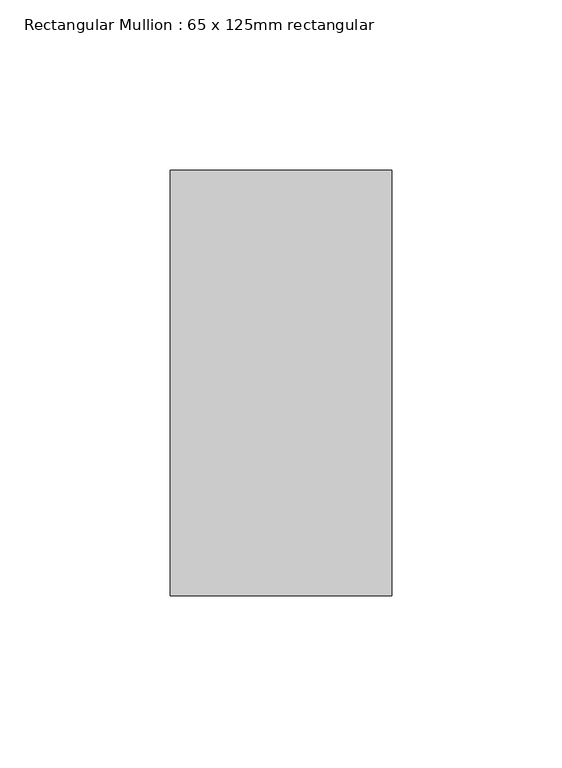
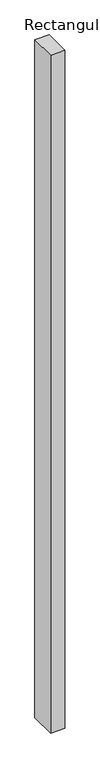
"""IFC4 building model written with IfcOpenShell, lengths in millimetres: member geometry, Rectangular Mullion : 65 x 125mm rectangular."""

from ifc_helpers import new_model, si_unit, frame, origin, place, context, project, spatial, polyline, outline, extrude, source, transform, mapped, element, save


def rectangular_mullion_65_x_125mm_rectangular_6bff5ffe(model_context):
    return source(origin(), model_context, "Body", "SweptSolid", [
        extrude(outline(polyline([(0.0, 62.5), (0.0, -62.5), (-65.0, -62.5), (-65.0, 62.5), (0.0, 62.5)])), frame((0.0, 0.0, -3300.0), z_axis=(0.0, 0.0, 1.0), x_axis=(1.0, 0.0, 0.0)), (0.0, 0.0, 1.0), 3300.0),
    ])


if __name__ == "__main__":
    model = new_model("IFC4")
    model_context = context("Model", 3, world=origin())
    ifc_project = project(units=[si_unit("LENGTHUNIT", "METRE", prefix="MILLI")], contexts=[model_context])
    site = spatial("IfcSite", under=ifc_project)
    building = spatial("IfcBuilding", under=site)
    placement = place(None, origin())
    rectangular_mullion_65_x_125mm_rectangular_shape = rectangular_mullion_65_x_125mm_rectangular_6bff5ffe(model_context)
    element("IfcMember", 1, ObjectType="Rectangular Mullion : 65 x 125mm rectangular", at=placement, inside=building, context=model_context, shape_type="MappedRepresentation", body=[
        mapped(rectangular_mullion_65_x_125mm_rectangular_shape, transform((0.0, 0.0, 0.0), x_axis=(1.0, 0.0, 0.0), y_axis=(0.0, 1.0, 0.0), z_axis=(0.0, 0.0, 1.0))),
    ])
    save(model, "model.ifc")

# Revit data of these elements
# Type "Rectangular Mullion : 65 x 125mm rectangular"
#   built-in parameter 1007304 = 0.410105 (stored number, unit not read)
#   built-in parameter 1007301 = 0.106627 (stored number, unit not read)
#   built-in parameter 1007300 = 0.106627 (stored number, unit not read)
# Element 1 (IfcMember, "Rectangular Mullion : 65 x 125mm rectangular")
#   Materials on its faces: "Aluminum"
# Materials
#   "Aluminum": class "Metal", colour RGB 244 245 246, transparency 0, Description = "Aluminum 6061", Cost = 0
